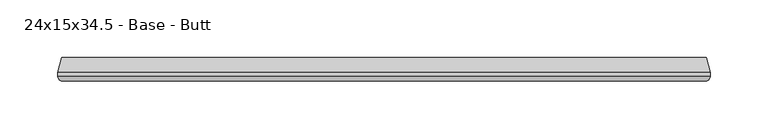
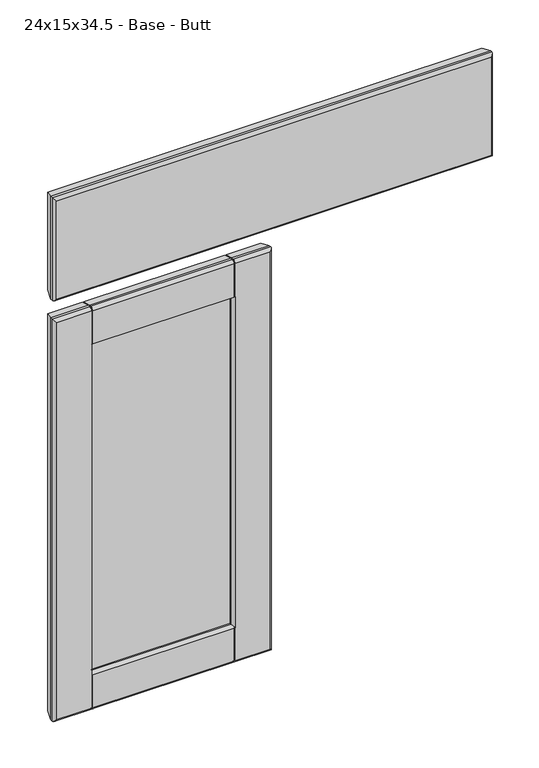
"""IFC4 building model written with IfcOpenShell, lengths in millimetres: furniture geometry, Cabinet-Base-Merillat-Double_Door-Marlin : 24x15x34.5 - Base - Butt."""

from ifc_helpers import new_model, si_unit, frame, origin, place, context, project, spatial, polyline, circle_curve, ellipse_curve, outline, extrude, source, transform, mapped, element, save
from ifc_brep_helpers import plane_surface, cylinder_surface, advanced_brep


def furniture_24x15x34_5_base_butt_84ca6513(model_context):
    return source(origin(), model_context, "Body", "SolidModel", [
        advanced_brep(
        [(-260.7408026, -629.92, 847.8035075), (-260.7408026, -629.92, 714.2964925), (298.2162124, -629.92, 714.2964925), (298.2162124, -629.92, 847.8035075), (-260.3320951, -609.6, 714.7052), (-260.3320951, -609.6, 847.3948), (297.8075049, -609.6, 847.3948), (297.8075049, -609.6, 714.7052), (-263.8372951, -625.4496, 850.9), (-263.8372951, -622.681, 850.9), (-263.8372951, -622.681, 711.2), (-263.8372951, -625.4496, 711.2), (301.3127049, -622.681, 711.2), (301.3127049, -625.4496, 711.2), (301.3127049, -622.681, 850.9), (301.3127049, -625.4496, 850.9)],
        [
            (0, 1),
            (1, 2),
            (2, 3),
            (3, 0),
            (4, 5),
            (5, 6),
            (6, 7),
            (7, 4),
            (8, 9),
            (9, 10),
            (10, 11),
            (11, 8),
            (10, 12),
            (12, 13),
            (13, 11),
            (12, 14),
            (14, 15),
            (15, 13),
            (8, 15),
            (14, 9),
            (11, 1, ellipse_curve(frame((-259.0620951, -625.4496, 715.9752), z_axis=(-0.7071067811865475, 0.0, 0.7071067811865475), x_axis=(-0.7071067811865474, 0.0, -0.7071067811865476)), 6.7531526, 4.7752)),
            (0, 8, ellipse_curve(frame((-259.0620951, -625.4496, 846.1248), z_axis=(-0.7071067811865475, 0.0, -0.7071067811865475), x_axis=(0.7071067811865474, 0.0, -0.7071067811865476)), 6.7531526, 4.7752)),
            (4, 10),
            (9, 5),
            (13, 2, ellipse_curve(frame((296.5375049, -625.4496, 715.9752), z_axis=(-0.7071067811865475, 0.0, -0.7071067811865475), x_axis=(0.7071067811865476, 0.0, -0.7071067811865474)), 6.7531526, 4.7752)),
            (7, 12),
            (15, 3, ellipse_curve(frame((296.5375049, -625.4496, 846.1248), z_axis=(0.7071067811865475, 0.0, -0.7071067811865475), x_axis=(0.7071067811865474, 0.0, 0.7071067811865476)), 6.7531526, 4.7752)),
            (6, 14),
        ],
        [
            plane_surface(frame((-263.8372951, -629.92, 850.9), z_axis=(0.0, -1.0, 0.0), x_axis=(0.0, 0.0, -1.0))),
            plane_surface(frame((-263.8372951, -609.6, 850.9), z_axis=(0.0, 1.0, 0.0), x_axis=(0.0, 0.0, 1.0))),
            plane_surface(frame((-263.8372951, -629.92, 850.9), z_axis=(-1.0, 0.0, 0.0), x_axis=(0.0, 1.0, 0.0))),
            plane_surface(frame((-263.8372951, -629.92, 711.2), z_axis=(0.0, 0.0, -1.0), x_axis=(0.0, 1.0, 0.0))),
            plane_surface(frame((301.3127049, -629.92, 711.2), z_axis=(1.0, 0.0, 0.0), x_axis=(0.0, 1.0, 0.0))),
            plane_surface(frame((301.3127049, -629.92, 850.9), z_axis=(0.0, 0.0, 1.0), x_axis=(0.0, 1.0, 0.0))),
            cylinder_surface(frame((-259.0620951, -625.4496, 850.9), z_axis=(0.0, 0.0, -1.0), x_axis=(0.0, 1.0, 0.0)), 4.7752),
            plane_surface(frame((-263.8372951, -622.681, 850.9), z_axis=(-0.9659229350723619, 0.25882983502910506, 0.0), x_axis=(0.0, 0.0, -1.0))),
            cylinder_surface(frame((-263.8372951, -625.4496, 715.9752), z_axis=(1.0, 0.0, 0.0), x_axis=(0.0, 1.0, 0.0)), 4.7752),
            plane_surface(frame((-263.8372951, -622.681, 711.2), z_axis=(0.0, 0.25882983502910506, -0.9659229350723619), x_axis=(1.0, 0.0, 0.0))),
            cylinder_surface(frame((296.5375049, -625.4496, 711.2), z_axis=(0.0, 0.0, 1.0), x_axis=(0.0, 1.0, 0.0)), 4.7752),
            plane_surface(frame((301.3127049, -622.681, 711.2), z_axis=(0.9659229350723619, 0.25882983502910506, 0.0), x_axis=(0.0, 0.0, 1.0))),
            cylinder_surface(frame((301.3127049, -625.4496, 846.1248), z_axis=(-1.0, 0.0, 0.0), x_axis=(0.0, 1.0, 0.0)), 4.7752),
            plane_surface(frame((301.3127049, -622.681, 850.9), z_axis=(0.0, 0.25882983502910506, 0.9659229350723619), x_axis=(-1.0, 0.0, 0.0))),
        ],
        [
            (0, [[1, 2, 3, 4]]),
            (1, [[5, 6, 7, 8]]),
            (2, [[9, 10, 11, 12]]),
            (3, [[-11, 13, 14, 15]]),
            (4, [[-14, 16, 17, 18]]),
            (5, [[-9, 19, -17, 20]]),
            (6, [[21, -1, 22, -12]]),
            (7, [[23, -10, 24, -5]]),
            (8, [[-21, -15, 25, -2]]),
            (9, [[-23, -8, 26, -13]]),
            (10, [[-25, -18, 27, -3]]),
            (11, [[-26, -7, 28, -16]]),
            (12, [[-22, -4, -27, -19]]),
            (13, [[-24, -20, -28, -6]]),
        ],
    ),
        advanced_brep(
        [(-263.8372951, -625.4496, 685.8), (-263.8372951, -625.4496, 139.7), (-260.7408026, -629.92, 142.7964925), (-260.7408026, -629.92, 682.7035075), (-263.8372951, -622.681, 685.8), (-263.8372951, -622.681, 139.7), (-260.3320951, -609.6, 682.2948), (-260.3320951, -609.6, 143.2052), (-215.6361323, -609.6, 637.5988372), (-215.2660006, -610.39375, 637.2287055), (-213.1848416, -614.85681, 635.1475465), (-213.1848416, -614.85681, 190.3524535), (-215.2660006, -610.39375, 188.2712945), (-215.6361323, -609.6, 187.9011628), (-214.584611, -617.0969093, 636.547316), (-214.584611, -617.0969093, 188.952684), (-228.9122951, -617.347, 650.875), (-228.9122951, -617.347, 174.625), (-228.9122951, -622.173, 650.875), (-228.9122951, -622.173, 174.625), (-214.584611, -622.4230907, 636.547316), (-214.584611, -622.4230907, 188.952684), (-213.1848416, -624.66319, 635.1475465), (-213.1848416, -624.66319, 190.3524535), (-215.2660006, -629.12625, 637.2287055), (-215.6332649, -629.9138508, 637.5959698), (-215.6361323, -629.92, 187.9011628), (-215.2660006, -629.12625, 188.2712945), (14.0537124, -629.92, 142.7964925), (-31.0140137, -629.92, 142.7964925), (-31.0140137, -625.4496, 139.7), (17.1502049, -625.4496, 139.7), (-215.6332649, -625.4496, 139.7), (-215.6332649, -629.92, 142.7964925), (-214.0457649, -625.4496, 139.7), (-32.6015137, -625.4496, 139.7), (-32.6015137, -629.92, 142.7964925), (-214.0457649, -629.92, 142.7964925), (-31.0140137, -622.681, 139.7), (17.1502049, -622.681, 139.7), (-215.6332649, -622.681, 139.7), (-214.0457649, -622.681, 139.7), (-32.6015137, -622.681, 139.7), (-31.0140137, -609.6, 143.2052), (13.6450049, -609.6, 143.2052), (-214.0457649, -609.6, 143.2052), (-32.6015137, -609.6, 143.2052), (-215.6332649, -609.6, 143.2052), (-33.5022486, -614.85681, 190.3524535), (-31.4210895, -610.39375, 188.2712945), (-32.6015137, -610.39375, 188.2712945), (-32.6015137, -609.6, 187.9011628), (-214.0457649, -609.6, 187.9011628), (-214.0457649, -610.39375, 188.2712945), (-32.1024791, -617.0969093, 188.952684), (-17.7747951, -617.347, 174.625), (-17.7747951, -622.173, 174.625), (-32.1024791, -622.4230907, 188.952684), (-33.5022486, -624.66319, 190.3524535), (-214.0457649, -629.12625, 188.2712945), (-214.0457649, -629.92, 187.9011628), (-32.6015137, -629.92, 187.9011628), (-32.6015137, -629.12625, 188.2712945), (-31.4210895, -629.12625, 188.2712945), (17.1502049, -625.4496, 685.8), (14.0537124, -629.92, 682.7035075), (17.1502049, -622.681, 685.8), (13.6450049, -609.6, 682.2948), (-31.0509578, -609.6, 187.9011628), (-33.5022486, -614.85681, 635.1475465), (-31.4210895, -610.39375, 637.2287055), (-31.0509578, -609.6, 637.5988372), (-32.1024791, -617.0969093, 636.547316), (-17.7747951, -617.347, 650.875), (-17.7747951, -622.173, 650.875), (-32.1024791, -622.4230907, 636.547316), (-33.5022486, -624.66319, 635.1475465), (-31.0509578, -629.92, 187.9011628), (-31.0509578, -629.92, 637.5988372), (-31.4210895, -629.12625, 637.2287055), (-215.6332649, -629.92, 682.7035075), (-215.6332649, -625.4496, 685.8), (-31.0140137, -625.4496, 685.8), (-31.0140137, -629.92, 682.7035075), (-32.6015137, -625.4496, 685.8), (-214.0457649, -625.4496, 685.8), (-214.0457649, -629.92, 682.7035075), (-32.6015137, -629.92, 682.7035075), (-215.6332649, -622.681, 685.8), (-31.0140137, -622.681, 685.8), (-32.6015137, -622.681, 685.8), (-214.0457649, -622.681, 685.8), (-215.6332649, -609.6, 682.2948), (-31.0140137, -609.6, 682.2948), (-32.6015137, -609.6, 682.2948), (-214.0457649, -609.6, 682.2948), (-32.6015137, -609.6, 637.5988372), (-214.0457649, -609.6, 637.5988372), (-214.0457649, -610.39375, 637.2287055), (-32.6015137, -610.39375, 637.2287055), (-32.6015137, -629.12625, 637.2287055), (-32.6015137, -629.92, 637.5988372), (-214.0457649, -629.92, 637.5988372), (-214.0457649, -629.12625, 637.2287055), (-32.6015137, -629.12625, 682.5526052), (-32.6015137, -625.4496, 685.00625), (-32.6015137, -622.7855037, 685.00625), (-32.6015137, -610.39375, 681.6857412), (-31.0140137, -610.39375, 637.2287055), (-31.0140137, -610.39375, 681.6857412), (-31.0140137, -622.7855037, 685.00625), (-31.0140137, -625.4496, 685.00625), (-31.0140137, -629.12625, 682.5526052), (-31.0140137, -629.12625, 637.2287055), (-215.6332649, -629.12625, 637.2287055), (-215.6332649, -629.12625, 682.5526052), (-215.6332649, -625.4496, 685.00625), (-215.6332649, -622.7855037, 685.00625), (-215.6332649, -610.39375, 681.6857412), (-215.6332649, -610.39375, 637.2287055), (-214.0457649, -610.39375, 681.6857412), (-214.0457649, -622.7855037, 685.00625), (-214.0457649, -625.4496, 685.00625), (-214.0457649, -629.12625, 682.5526052), (-215.6332649, -610.39375, 188.2712945), (-215.6332649, -610.39375, 143.8142588), (-215.6332649, -622.7855037, 140.49375), (-215.6332649, -625.4496, 140.49375), (-215.6332649, -629.12625, 142.9473948), (-215.6332649, -629.12625, 188.2712945), (-214.0457649, -629.12625, 142.9473948), (-214.0457649, -625.4496, 140.49375), (-214.0457649, -622.7855037, 140.49375), (-214.0457649, -610.39375, 143.8142588), (-32.6015137, -610.39375, 143.8142588), (-32.6015137, -622.7855037, 140.49375), (-32.6015137, -625.4496, 140.49375), (-32.6015137, -629.12625, 142.9473948), (-31.0140137, -629.12625, 188.2712945), (-31.0140137, -629.12625, 142.9473948), (-31.0140137, -625.4496, 140.49375), (-31.0140137, -622.7855037, 140.49375), (-31.0140137, -610.39375, 143.8142588), (-31.0140137, -610.39375, 188.2712945)],
        [
            (0, 1),
            (1, 2, ellipse_curve(frame((-259.0620951, -625.4496, 144.4752), z_axis=(-0.7071067811865475, 0.0, 0.7071067811865475), x_axis=(0.7071067811865474, 0.0, 0.7071067811865476)), 6.7531526, 4.7752)),
            (2, 3),
            (3, 0, ellipse_curve(frame((-259.0620951, -625.4496, 681.0248), z_axis=(-0.7071067811865475, 0.0, -0.7071067811865475), x_axis=(-0.7071067811865474, 0.0, 0.7071067811865476)), 6.7531526, 4.7752)),
            (0, 4),
            (4, 5),
            (5, 1),
            (4, 6),
            (6, 7),
            (7, 5),
            (8, 9),
            (9, 10),
            (10, 11),
            (11, 12),
            (12, 13),
            (13, 8),
            (10, 14, ellipse_curve(frame((-214.6120951, -615.5223492, 636.5748), z_axis=(-0.7071067811865475, 0.0, -0.7071067811865475), x_axis=(-0.7071067811865474, 0.0, 0.7071067811865476)), 2.2271035, 1.5748)),
            (14, 15),
            (15, 11, ellipse_curve(frame((-214.6120951, -615.5223492, 188.9252), z_axis=(-0.7071067811865475, 0.0, 0.7071067811865475), x_axis=(0.7071067811865474, 0.0, 0.7071067811865476)), 2.2271035, 1.5748)),
            (14, 16),
            (16, 17),
            (17, 15),
            (16, 18),
            (18, 19),
            (19, 17),
            (18, 20),
            (20, 21),
            (21, 19),
            (20, 22, ellipse_curve(frame((-214.6120951, -623.9976508, 636.5748), z_axis=(-0.7071067811865475, 0.0, -0.7071067811865475), x_axis=(-0.7071067811865474, 0.0, 0.7071067811865476)), 2.2271035, 1.5748)),
            (22, 23),
            (23, 21, ellipse_curve(frame((-214.6120951, -623.9976508, 188.9252), z_axis=(-0.7071067811865475, 0.0, 0.7071067811865475), x_axis=(0.7071067811865474, 0.0, 0.7071067811865476)), 2.2271035, 1.5748)),
            (22, 24),
            (24, 25),
            (25, 26),
            (26, 27),
            (27, 23),
            (28, 29),
            (29, 30, circle_curve(frame((-31.0140137, -625.4496, 144.4752), z_axis=(1.0, 0.0, 0.0), x_axis=(0.0, 1.0, 0.0)), 4.7752)),
            (30, 31),
            (31, 28, ellipse_curve(frame((12.3750049, -625.4496, 144.4752), z_axis=(-0.7071067811865475, 0.0, -0.7071067811865475), x_axis=(-0.7071067811865476, 0.0, 0.7071067811865474)), 6.7531526, 4.7752)),
            (1, 32),
            (32, 33, circle_curve(frame((-215.6332649, -625.4496, 144.4752), z_axis=(-1.0, 0.0, 0.0), x_axis=(0.0, 1.0, 0.0)), 4.7752)),
            (33, 2),
            (34, 35),
            (35, 36, circle_curve(frame((-32.6015137, -625.4496, 144.4752), z_axis=(-1.0, 0.0, 0.0), x_axis=(0.0, 1.0, 0.0)), 4.7752)),
            (36, 37),
            (37, 34, circle_curve(frame((-214.0457649, -625.4496, 144.4752), z_axis=(1.0, 0.0, 0.0), x_axis=(0.0, 1.0, 0.0)), 4.7752)),
            (30, 38),
            (38, 39),
            (39, 31),
            (5, 40),
            (40, 32),
            (41, 42),
            (42, 35),
            (34, 41),
            (38, 43),
            (43, 44),
            (44, 39),
            (45, 46),
            (46, 42),
            (41, 45),
            (7, 47),
            (47, 40),
            (48, 49),
            (49, 50),
            (50, 51),
            (51, 52),
            (52, 53),
            (53, 12),
            (11, 48),
            (15, 54),
            (54, 48, ellipse_curve(frame((-32.0749951, -615.5223492, 188.9252), z_axis=(-0.7071067811865475, 0.0, -0.7071067811865475), x_axis=(-0.7071067811865476, 0.0, 0.7071067811865474)), 2.2271035, 1.5748)),
            (17, 55),
            (55, 54),
            (19, 56),
            (56, 55),
            (21, 57),
            (57, 56),
            (23, 58),
            (58, 57, ellipse_curve(frame((-32.0749951, -623.9976508, 188.9252), z_axis=(-0.7071067811865475, 0.0, -0.7071067811865475), x_axis=(-0.7071067811865476, 0.0, 0.7071067811865474)), 2.2271035, 1.5748)),
            (27, 59),
            (59, 60),
            (60, 61),
            (61, 62),
            (62, 63),
            (63, 58),
            (31, 64),
            (64, 65, ellipse_curve(frame((12.3750049, -625.4496, 681.0248), z_axis=(0.7071067811865475, 0.0, -0.7071067811865475), x_axis=(-0.7071067811865474, 0.0, -0.7071067811865476)), 6.7531526, 4.7752)),
            (65, 28),
            (39, 66),
            (66, 64),
            (44, 67),
            (67, 66),
            (68, 49),
            (48, 69),
            (69, 70),
            (70, 71),
            (71, 68),
            (54, 72),
            (72, 69, ellipse_curve(frame((-32.0749951, -615.5223492, 636.5748), z_axis=(0.7071067811865475, 0.0, -0.7071067811865475), x_axis=(-0.7071067811865474, 0.0, -0.7071067811865476)), 2.2271035, 1.5748)),
            (55, 73),
            (73, 72),
            (56, 74),
            (74, 73),
            (57, 75),
            (75, 74),
            (58, 76),
            (76, 75, ellipse_curve(frame((-32.0749951, -623.9976508, 636.5748), z_axis=(0.7071067811865475, 0.0, -0.7071067811865475), x_axis=(-0.7071067811865474, 0.0, -0.7071067811865476)), 2.2271035, 1.5748)),
            (63, 77),
            (77, 78),
            (78, 79),
            (79, 76),
            (3, 80),
            (80, 81, circle_curve(frame((-215.6332649, -625.4496, 681.0248), z_axis=(-1.0, 0.0, 0.0), x_axis=(0.0, 1.0, 0.0)), 4.7752)),
            (81, 0),
            (64, 82),
            (82, 83, circle_curve(frame((-31.0140137, -625.4496, 681.0248), z_axis=(1.0, 0.0, 0.0), x_axis=(0.0, 1.0, 0.0)), 4.7752)),
            (83, 65),
            (84, 85),
            (85, 86, circle_curve(frame((-214.0457649, -625.4496, 681.0248), z_axis=(1.0, 0.0, 0.0), x_axis=(0.0, 1.0, 0.0)), 4.7752)),
            (86, 87),
            (87, 84, circle_curve(frame((-32.6015137, -625.4496, 681.0248), z_axis=(-1.0, 0.0, 0.0), x_axis=(0.0, 1.0, 0.0)), 4.7752)),
            (81, 88),
            (88, 4),
            (66, 89),
            (89, 82),
            (90, 91),
            (91, 85),
            (84, 90),
            (88, 92),
            (92, 6),
            (67, 93),
            (93, 89),
            (94, 95),
            (95, 91),
            (90, 94),
            (51, 46),
            (45, 52),
            (43, 68),
            (71, 93),
            (92, 8),
            (13, 47),
            (96, 97),
            (97, 95),
            (94, 96),
            (9, 98),
            (98, 97),
            (96, 99),
            (99, 70),
            (69, 10),
            (72, 14),
            (73, 16),
            (74, 18),
            (75, 20),
            (76, 22),
            (79, 100),
            (100, 101),
            (101, 102),
            (102, 103),
            (103, 24),
            (33, 26),
            (25, 80),
            (36, 61),
            (60, 37),
            (83, 78),
            (77, 29),
            (86, 102),
            (101, 87),
            (100, 104),
            (104, 105, circle_curve(frame((-32.6015137, -625.4496, 681.0248), z_axis=(-1.0, 0.0, 0.0), x_axis=(0.0, 0.0, 1.0)), 3.98145)),
            (105, 106),
            (106, 107),
            (107, 99),
            (71, 108),
            (108, 109),
            (109, 110),
            (110, 111),
            (111, 112, circle_curve(frame((-31.0140137, -625.4496, 681.0248), z_axis=(1.0, 0.0, 0.0), x_axis=(0.0, 0.0, 1.0)), 3.98145)),
            (112, 113),
            (113, 78),
            (113, 79),
            (112, 104),
            (111, 105),
            (110, 106),
            (109, 107),
            (108, 70),
            (25, 114),
            (114, 115),
            (115, 116, circle_curve(frame((-215.6332649, -625.4496, 681.0248), z_axis=(-1.0, 0.0, 0.0), x_axis=(0.0, 0.0, 1.0)), 3.98145)),
            (116, 117),
            (117, 118),
            (118, 119),
            (119, 8),
            (98, 120),
            (120, 121),
            (121, 122),
            (122, 123, circle_curve(frame((-214.0457649, -625.4496, 681.0248), z_axis=(1.0, 0.0, 0.0), x_axis=(0.0, 0.0, 1.0)), 3.98145)),
            (123, 103),
            (24, 114),
            (123, 115),
            (122, 116),
            (121, 117),
            (120, 118),
            (9, 119),
            (13, 124),
            (124, 125),
            (125, 126),
            (126, 127),
            (127, 128, circle_curve(frame((-215.6332649, -625.4496, 144.4752), z_axis=(-1.0, 0.0, 0.0), x_axis=(0.0, 0.0, 1.0)), 3.98145)),
            (128, 129),
            (129, 26),
            (59, 130),
            (130, 131, circle_curve(frame((-214.0457649, -625.4496, 144.4752), z_axis=(1.0, 0.0, 0.0), x_axis=(0.0, 0.0, 1.0)), 3.98145)),
            (131, 132),
            (132, 133),
            (133, 53),
            (12, 124),
            (133, 125),
            (132, 126),
            (131, 127),
            (130, 128),
            (27, 129),
            (50, 134),
            (134, 135),
            (135, 136),
            (136, 137, circle_curve(frame((-32.6015137, -625.4496, 144.4752), z_axis=(-1.0, 0.0, 0.0), x_axis=(0.0, 0.0, 1.0)), 3.98145)),
            (137, 62),
            (138, 139),
            (139, 140, circle_curve(frame((-31.0140137, -625.4496, 144.4752), z_axis=(1.0, 0.0, 0.0), x_axis=(0.0, 0.0, 1.0)), 3.98145)),
            (140, 141),
            (141, 142),
            (142, 143),
            (143, 68),
            (77, 138),
            (63, 138),
            (143, 49),
            (142, 134),
            (141, 135),
            (140, 136),
            (139, 137),
        ],
        [
            cylinder_surface(frame((-259.0620951, -625.4496, 685.8), z_axis=(0.0, 0.0, 1.0), x_axis=(0.0, 1.0, 0.0)), 4.7752),
            plane_surface(frame((-263.8372951, -625.4496, 685.8), z_axis=(-1.0, 0.0, 0.0), x_axis=(0.0, 0.0, -1.0))),
            plane_surface(frame((-263.8372951, -622.681, 685.8), z_axis=(-0.9659229350723619, 0.25882983502910506, 0.0), x_axis=(0.0, 0.0, -1.0))),
            plane_surface(frame((-215.6361323, -609.6, 637.5988372), z_axis=(0.9063077870366099, 0.4226182617407856, 0.0), x_axis=(0.0, 0.0, -1.0))),
            cylinder_surface(frame((-214.6120951, -615.5223492, 685.8), z_axis=(0.0, 0.0, 1.0000000000000002), x_axis=(0.01745240643729364, -0.9998476951563912, 0.0)), 1.5748),
            plane_surface(frame((-214.584611, -617.0969093, 636.547316), z_axis=(0.017452406437322144, -0.9998476951563906, 0.0), x_axis=(0.0, 0.0, -1.0))),
            plane_surface(frame((-228.9122951, -617.347, 650.875), z_axis=(1.0, 0.0, 0.0), x_axis=(0.0, 0.0, -1.0))),
            plane_surface(frame((-228.9122951, -622.173, 650.875), z_axis=(0.01745240643727848, 0.9998476951563914, 0.0), x_axis=(0.0, 0.0, -1.0))),
            cylinder_surface(frame((-214.6120951, -623.9976508, 685.8), z_axis=(0.0, 0.0, 1.0000000000000002), x_axis=(0.9063077870367326, -0.42261826174052236, 0.0)), 1.5748),
            plane_surface(frame((-213.1848416, -624.66319, 635.1475465), z_axis=(0.9063077870366333, -0.4226182617407352, 0.0), x_axis=(0.0, 0.0, -1.0))),
            cylinder_surface(frame((-263.8372951, -625.4496, 144.4752), z_axis=(-1.0, 0.0, 0.0), x_axis=(0.0, 1.0, 0.0)), 4.7752),
            plane_surface(frame((-263.8372951, -625.4496, 139.7), z_axis=(0.0, 0.0, -1.0), x_axis=(1.0, 0.0, 0.0))),
            plane_surface(frame((-263.8372951, -622.681, 139.7), z_axis=(0.0, 0.25882983502910506, -0.9659229350723619), x_axis=(1.0, 0.0, 0.0))),
            plane_surface(frame((-215.6361323, -609.6, 187.9011628), z_axis=(0.0, 0.4226182617407856, 0.9063077870366099), x_axis=(1.0, 0.0, 0.0))),
            cylinder_surface(frame((-263.8372951, -615.5223492, 188.9252), z_axis=(-1.0000000000000002, 0.0, 0.0), x_axis=(0.0, -0.9998476951563912, 0.01745240643729364)), 1.5748),
            plane_surface(frame((-214.584611, -617.0969093, 188.952684), z_axis=(0.0, -0.9998476951563906, 0.017452406437322144), x_axis=(1.0, 0.0, 0.0))),
            plane_surface(frame((-228.9122951, -617.347, 174.625), z_axis=(0.0, 0.0, 1.0), x_axis=(1.0, 0.0, 0.0))),
            plane_surface(frame((-228.9122951, -622.173, 174.625), z_axis=(0.0, 0.9998476951563914, 0.01745240643727848), x_axis=(1.0, 0.0, 0.0))),
            cylinder_surface(frame((-263.8372951, -623.9976508, 188.9252), z_axis=(-1.0000000000000002, 0.0, 0.0), x_axis=(0.0, -0.42261826174052236, 0.9063077870367326)), 1.5748),
            plane_surface(frame((-213.1848416, -624.66319, 190.3524535), z_axis=(0.0, -0.4226182617407352, 0.9063077870366333), x_axis=(1.0, 0.0, 0.0))),
            cylinder_surface(frame((12.3750049, -625.4496, 139.7), z_axis=(0.0, 0.0, -1.0), x_axis=(0.0, 1.0, 0.0)), 4.7752),
            plane_surface(frame((17.1502049, -625.4496, 139.7), z_axis=(1.0, 0.0, 0.0), x_axis=(0.0, 0.0, 1.0))),
            plane_surface(frame((17.1502049, -622.681, 139.7), z_axis=(0.9659229350723619, 0.25882983502910506, 0.0), x_axis=(0.0, 0.0, 1.0))),
            plane_surface(frame((-31.0509578, -609.6, 187.9011628), z_axis=(-0.9063077870366099, 0.4226182617407856, 0.0), x_axis=(0.0, 0.0, 1.0))),
            cylinder_surface(frame((-32.0749951, -615.5223492, 139.7), z_axis=(0.0, 0.0, -1.0000000000000002), x_axis=(-0.01745240643729364, -0.9998476951563912, 0.0)), 1.5748),
            plane_surface(frame((-32.1024791, -617.0969093, 188.952684), z_axis=(-0.017452406437322144, -0.9998476951563906, 0.0), x_axis=(0.0, 0.0, 1.0))),
            plane_surface(frame((-17.7747951, -617.347, 174.625), z_axis=(-1.0, 0.0, 0.0), x_axis=(0.0, 0.0, 1.0))),
            plane_surface(frame((-17.7747951, -622.173, 174.625), z_axis=(-0.01745240643727848, 0.9998476951563914, 0.0), x_axis=(0.0, 0.0, 1.0))),
            cylinder_surface(frame((-32.0749951, -623.9976508, 139.7), z_axis=(0.0, 0.0, -1.0000000000000002), x_axis=(-0.9063077870367326, -0.42261826174052236, 0.0)), 1.5748),
            plane_surface(frame((-33.5022486, -624.66319, 190.3524535), z_axis=(-0.9063077870366333, -0.4226182617407352, 0.0), x_axis=(0.0, 0.0, 1.0))),
            cylinder_surface(frame((17.1502049, -625.4496, 681.0248), z_axis=(1.0, 0.0, 0.0), x_axis=(0.0, 1.0, 0.0)), 4.7752),
            plane_surface(frame((17.1502049, -625.4496, 685.8), z_axis=(0.0, 0.0, 1.0), x_axis=(-1.0, 0.0, 0.0))),
            plane_surface(frame((17.1502049, -622.681, 685.8), z_axis=(0.0, 0.25882983502910506, 0.9659229350723619), x_axis=(-1.0, 0.0, 0.0))),
            plane_surface(frame((13.6450049, -609.6, 682.2948), z_axis=(0.0, 1.0, 0.0), x_axis=(-1.0, 0.0, 0.0))),
            plane_surface(frame((-31.0509578, -609.6, 637.5988372), z_axis=(0.0, 0.4226182617407856, -0.9063077870366099), x_axis=(-1.0, 0.0, 0.0))),
            cylinder_surface(frame((17.1502049, -615.5223492, 636.5748), z_axis=(1.0000000000000002, 0.0, 0.0), x_axis=(0.0, -0.9998476951563912, -0.01745240643729364)), 1.5748),
            plane_surface(frame((-32.1024791, -617.0969093, 636.547316), z_axis=(0.0, -0.9998476951563906, -0.017452406437322144), x_axis=(-1.0, 0.0, 0.0))),
            plane_surface(frame((-17.7747951, -617.347, 650.875), z_axis=(0.0, 0.0, -1.0), x_axis=(-1.0, 0.0, 0.0))),
            plane_surface(frame((-17.7747951, -622.173, 650.875), z_axis=(0.0, 0.9998476951563914, -0.01745240643727848), x_axis=(-1.0, 0.0, 0.0))),
            cylinder_surface(frame((17.1502049, -623.9976508, 636.5748), z_axis=(1.0000000000000002, 0.0, 0.0), x_axis=(0.0, -0.42261826174052236, -0.9063077870367326)), 1.5748),
            plane_surface(frame((-33.5022486, -624.66319, 635.1475465), z_axis=(0.0, -0.4226182617407352, -0.9063077870366333), x_axis=(-1.0, 0.0, 0.0))),
            plane_surface(frame((-31.0509578, -629.92, 637.5988372), z_axis=(0.0, -1.0, 0.0), x_axis=(-1.0, 0.0, 0.0))),
            plane_surface(frame((-32.6015137, -629.92, 637.5988372), z_axis=(1.0, 0.0, 0.0), x_axis=(0.0, 0.906307787036771, -0.4226182617404399))),
            plane_surface(frame((-31.0140137, -629.92, 637.5988372), z_axis=(-1.0, 0.0, 0.0), x_axis=(0.0, -0.906307787036771, 0.4226182617404399))),
            plane_surface(frame((-32.6015137, -629.92, 637.5988372), z_axis=(0.0, 0.4226182617404399, 0.906307787036771), x_axis=(1.0, 0.0, 0.0))),
            plane_surface(frame((-32.6015137, -629.12625, 637.2287055), z_axis=(0.0, -1.0, 0.0), x_axis=(1.0, 0.0, 0.0))),
            cylinder_surface(frame((-31.0140137, -625.4496, 681.0248), z_axis=(1.0, 0.0, 0.0), x_axis=(0.0, 0.0, 1.0)), 3.98145),
            plane_surface(frame((-32.6015137, -625.4496, 685.00625), z_axis=(0.0, 0.0, 1.0), x_axis=(1.0, 0.0, 0.0))),
            plane_surface(frame((-32.6015137, -622.7855037, 685.00625), z_axis=(0.0, 0.25882983502913415, 0.9659229350723542), x_axis=(1.0, 0.0, 0.0))),
            plane_surface(frame((-32.6015137, -610.39375, 681.6857412), z_axis=(0.0, 1.0, 0.0), x_axis=(1.0, 0.0, 0.0))),
            plane_surface(frame((-32.6015137, -610.39375, 637.2287055), z_axis=(0.0, -0.4226182617405111, 0.9063077870367379), x_axis=(1.0, 0.0, 0.0))),
            plane_surface(frame((-215.6332649, -629.92, 637.5988372), z_axis=(1.0, 0.0, 0.0), x_axis=(0.0, 0.9063077870367783, -0.42261826174042444))),
            plane_surface(frame((-214.0457649, -629.92, 637.5988372), z_axis=(-1.0, 0.0, 0.0), x_axis=(0.0, -0.9063077870367783, 0.42261826174042444))),
            plane_surface(frame((-215.6332649, -629.92, 637.5988372), z_axis=(0.0, 0.42261826174042444, 0.9063077870367783), x_axis=(1.0, 0.0, 0.0))),
            plane_surface(frame((-215.6332649, -629.12625, 637.2287055), z_axis=(0.0, -1.0, 0.0), x_axis=(1.0, 0.0, 0.0))),
            cylinder_surface(frame((-214.0457649, -625.4496, 681.0248), z_axis=(1.0, 0.0, 0.0), x_axis=(0.0, 0.0, 1.0)), 3.98145),
            plane_surface(frame((-215.6332649, -625.4496, 685.00625), z_axis=(0.0, 0.0, 1.0), x_axis=(1.0, 0.0, 0.0))),
            plane_surface(frame((-215.6332649, -622.7855037, 685.00625), z_axis=(0.0, 0.25882983502911566, 0.965922935072359), x_axis=(1.0, 0.0, 0.0))),
            plane_surface(frame((-215.6332649, -610.39375, 681.6857412), z_axis=(0.0, 1.0, 0.0), x_axis=(1.0, 0.0, 0.0))),
            plane_surface(frame((-215.6332649, -610.39375, 637.2287055), z_axis=(0.0, -0.42261826174056427, 0.9063077870367131), x_axis=(1.0, 0.0, 0.0))),
            plane_surface(frame((-215.6332649, -625.4496, 149.2504), z_axis=(1.0, 0.0, 0.0), x_axis=(0.0, -1.0, 0.0))),
            plane_surface(frame((-214.0457649, -625.4496, 149.2504), z_axis=(-1.0, 0.0, 0.0), x_axis=(0.0, 1.0, 0.0))),
            plane_surface(frame((-215.6332649, -609.6, 187.9011628), z_axis=(0.0, -0.42261826173999295, -0.9063077870369795), x_axis=(1.0, 0.0, 0.0))),
            plane_surface(frame((-215.6332649, -610.39375, 188.2712945), z_axis=(0.0, 1.0, 0.0), x_axis=(1.0, 0.0, 0.0))),
            plane_surface(frame((-215.6332649, -610.39375, 143.8142588), z_axis=(0.0, 0.2588298350290845, -0.9659229350723675), x_axis=(1.0, 0.0, 0.0))),
            plane_surface(frame((-215.6332649, -622.7855037, 140.49375), z_axis=(0.0, 0.0, -1.0), x_axis=(1.0, 0.0, 0.0))),
            cylinder_surface(frame((-214.0457649, -625.4496, 144.4752), z_axis=(1.0, 0.0, 0.0), x_axis=(0.0, 0.0, 1.0)), 3.98145),
            plane_surface(frame((-215.6332649, -629.12625, 142.9473948), z_axis=(0.0, -1.0, 0.0), x_axis=(1.0, 0.0, 0.0))),
            plane_surface(frame((-215.6332649, -629.12625, 188.2712945), z_axis=(0.0, 0.4226182617407698, -0.9063077870366172), x_axis=(1.0, 0.0, 0.0))),
            plane_surface(frame((-32.6015137, -629.12625, 188.2712945), z_axis=(1.0, 0.0, 0.0), x_axis=(0.0, -0.906307787036583, -0.42261826174084305))),
            plane_surface(frame((-31.0140137, -629.12625, 188.2712945), z_axis=(-1.0, 0.0, 0.0), x_axis=(0.0, 0.906307787036583, 0.42261826174084305))),
            plane_surface(frame((-32.6015137, -629.12625, 188.2712945), z_axis=(0.0, 0.42261826174084305, -0.906307787036583), x_axis=(1.0, 0.0, 0.0))),
            plane_surface(frame((-32.6015137, -609.6, 187.9011628), z_axis=(0.0, -0.42261826174073325, -0.9063077870366342), x_axis=(1.0, 0.0, 0.0))),
            plane_surface(frame((-32.6015137, -610.39375, 188.2712945), z_axis=(0.0, 1.0, 0.0), x_axis=(1.0, 0.0, 0.0))),
            plane_surface(frame((-32.6015137, -610.39375, 143.8142588), z_axis=(0.0, 0.2588298350290967, -0.9659229350723642), x_axis=(1.0, 0.0, 0.0))),
            plane_surface(frame((-32.6015137, -622.7855037, 140.49375), z_axis=(0.0, 0.0, -1.0), x_axis=(1.0, 0.0, 0.0))),
            cylinder_surface(frame((-31.0140137, -625.4496, 144.4752), z_axis=(1.0, 0.0, 0.0), x_axis=(0.0, 0.0, 1.0)), 3.98145),
            plane_surface(frame((-32.6015137, -629.12625, 142.9473948), z_axis=(0.0, -1.0, 0.0), x_axis=(1.0, 0.0, 0.0))),
        ],
        [
            (0, [[1, 2, 3, 4]]),
            (1, [[5, 6, 7, -1]]),
            (2, [[8, 9, 10, -6]]),
            (3, [[11, 12, 13, 14, 15, 16]]),
            (4, [[17, 18, 19, -13]]),
            (5, [[20, 21, 22, -18]]),
            (6, [[23, 24, 25, -21]]),
            (7, [[26, 27, 28, -24]]),
            (8, [[29, 30, 31, -27]]),
            (9, [[32, 33, 34, 35, 36, -30]]),
            (10, [[37, 38, 39, 40]]),
            (10, [[41, 42, 43, -2]]),
            (10, [[44, 45, 46, 47]]),
            (11, [[-39, 48, 49, 50]]),
            (11, [[51, 52, -41, -7]]),
            (11, [[53, 54, -44, 55]]),
            (12, [[-49, 56, 57, 58]]),
            (12, [[59, 60, -53, 61]]),
            (12, [[62, 63, -51, -10]]),
            (13, [[64, 65, 66, 67, 68, 69, -14, 70]]),
            (14, [[71, 72, -70, -19]]),
            (15, [[73, 74, -71, -22]]),
            (16, [[75, 76, -73, -25]]),
            (17, [[77, 78, -75, -28]]),
            (18, [[79, 80, -77, -31]]),
            (19, [[-36, 81, 82, 83, 84, 85, 86, -79]]),
            (20, [[87, 88, 89, -40]]),
            (21, [[90, 91, -87, -50]]),
            (22, [[92, 93, -90, -58]]),
            (23, [[94, -64, 95, 96, 97, 98]]),
            (24, [[99, 100, -95, -72]]),
            (25, [[101, 102, -99, -74]]),
            (26, [[103, 104, -101, -76]]),
            (27, [[105, 106, -103, -78]]),
            (28, [[107, 108, -105, -80]]),
            (29, [[-86, 109, 110, 111, 112, -107]]),
            (30, [[113, 114, 115, -4]]),
            (30, [[116, 117, 118, -88]]),
            (30, [[119, 120, 121, 122]]),
            (31, [[-115, 123, 124, -5]]),
            (31, [[125, 126, -116, -91]]),
            (31, [[127, 128, -119, 129]]),
            (32, [[-124, 130, 131, -8]]),
            (32, [[132, 133, -125, -93]]),
            (32, [[134, 135, -127, 136]]),
            (33, [[-67, 137, -59, 138]]),
            (33, [[-57, 139, -98, 140, -132, -92]]),
            (33, [[-131, 141, -16, 142, -62, -9]]),
            (33, [[143, 144, -134, 145]]),
            (34, [[-12, 146, 147, -143, 148, 149, -96, 150]]),
            (35, [[-150, -100, 151, -17]]),
            (36, [[-151, -102, 152, -20]]),
            (37, [[-152, -104, 153, -23]]),
            (38, [[-153, -106, 154, -26]]),
            (39, [[-154, -108, 155, -29]]),
            (40, [[-112, 156, 157, 158, 159, 160, -32, -155]]),
            (41, [[-43, 161, -34, 162, -113, -3]]),
            (41, [[-46, 163, -83, 164]]),
            (41, [[-118, 165, -110, 166, -37, -89]]),
            (41, [[-121, 167, -158, 168]]),
            (42, [[-148, -145, -136, -129, -122, -168, -157, 169, 170, 171, 172, 173]]),
            (43, [[-165, -117, -126, -133, -140, 174, 175, 176, 177, 178, 179, 180]]),
            (44, [[181, -111, -180]]),
            (45, [[-156, -181, -179, 182, -169]]),
            (46, [[-182, -178, 183, -170]]),
            (47, [[-183, -177, 184, -171]]),
            (48, [[-184, -176, 185, -172]]),
            (49, [[-185, -175, 186, -149, -173]]),
            (50, [[-97, -186, -174]]),
            (51, [[-141, -130, -123, -114, -162, 187, 188, 189, 190, 191, 192, 193]]),
            (52, [[-159, -167, -120, -128, -135, -144, -147, 194, 195, 196, 197, 198]]),
            (53, [[-33, 199, -187]]),
            (54, [[-199, -160, -198, 200, -188]]),
            (55, [[-200, -197, 201, -189]]),
            (56, [[-201, -196, 202, -190]]),
            (57, [[-202, -195, 203, -191]]),
            (58, [[-203, -194, -146, 204, -192]]),
            (59, [[-204, -11, -193]]),
            (60, [[-161, -42, -52, -63, -142, 205, 206, 207, 208, 209, 210, 211]]),
            (61, [[-68, -138, -61, -55, -47, -164, -82, 212, 213, 214, 215, 216]]),
            (62, [[-15, 217, -205]]),
            (63, [[-217, -69, -216, 218, -206]]),
            (64, [[-218, -215, 219, -207]]),
            (65, [[-219, -214, 220, -208]]),
            (66, [[-220, -213, 221, -209]]),
            (67, [[-221, -212, -81, 222, -210]]),
            (68, [[-222, -35, -211]]),
            (69, [[-84, -163, -45, -54, -60, -137, -66, 223, 224, 225, 226, 227]]),
            (70, [[228, 229, 230, 231, 232, 233, -139, -56, -48, -38, -166, 234]]),
            (71, [[-109, 235, -234]]),
            (72, [[236, -94, -233]]),
            (73, [[-65, -236, -232, 237, -223]]),
            (74, [[-237, -231, 238, -224]]),
            (75, [[-238, -230, 239, -225]]),
            (76, [[-239, -229, 240, -226]]),
            (77, [[-240, -228, -235, -85, -227]]),
        ],
    ),
        extrude(outline(polyline([(-17.7747951, -622.173), (-228.9122951, -622.173), (-228.9122951, -617.347), (-17.7747951, -617.347), (-17.7747951, -622.173)])), frame((0.0, 0.0, 174.625), z_axis=(0.0, 0.0, 1.0), x_axis=(1.0, 0.0, 0.0)), (0.0, 0.0, 1.0), 476.25),
    ])


if __name__ == "__main__":
    model = new_model("IFC4")
    model_context = context("Model", 3, world=origin())
    ifc_project = project(units=[si_unit("LENGTHUNIT", "METRE", prefix="MILLI")], contexts=[model_context])
    site = spatial("IfcSite", under=ifc_project)
    building = spatial("IfcBuilding", under=site)
    placement = place(None, origin())
    furniture_24x15x34_5_base_butt_shape = furniture_24x15x34_5_base_butt_84ca6513(model_context)
    element("IfcFurniture", 1, ObjectType="Cabinet-Base-Merillat-Double_Door-Marlin : 24x15x34.5 - Base - Butt", at=placement, inside=building, context=model_context, shape_type="MappedRepresentation", body=[
        mapped(furniture_24x15x34_5_base_butt_shape, transform((0.0, 0.0, 0.0), x_axis=(1.0, 0.0, 0.0), y_axis=(0.0, 1.0, 0.0), z_axis=(0.0, 0.0, 1.0))),
    ])
    save(model, "model.ifc")

# Revit data of these elements
# Type "Cabinet-Base-Merillat-Double_Door-Marlin : 24x15x34.5 - Base - Butt"
#   URL = "http://www.merillat.com"
#   Toe Kick Note = "Toe Kick Covering is not included. To be purchased Separately."
#   Product Line = "Express"
#   Product Page URL = "http://www.merillat.com//our-products/rooms/kitchen"
#   Product Group = "Base Cabinet"
#   Product Documentation Link = "http://merillatbusiness.com/customer-resources/product-line-resources/merillat-classic/"
#   Model = "B24B"
#   Manufacturer = "Merillat"
#   Finish = "Wood"
#   Description = "Base Butt Door"
#   Construction Type = "Deep Sink Base"
#   Cabinet Construction Note = "BUTT doors without a center frame stile, For tray or shelf option,  replace HDS with the option code of your choice,  When depth is reduced  to 12\" or 15\" drawer becomes false front"
#   Assembly Code = "C1030410"
#   Toe Kick Height = 0' - 4 1/2"
#   Toe Kick Depth = 0' - 2 25/32"
#   Top and Bottom Spacing = 0' - 1"
#   Side Spacing = 0' - 0 7/8"
#   Cabinet Shell = 0' - 0 3/8"
#   Door Spacing = 0' - 0 1/8"
#   Depth = 1' - 3"
#   Height = 2' - 10 1/2"
#   Width = 2' - 0"
#   Cabinet Drawer Width = 1' - 10 1/4"
#   Cabinet Drawer Height = 0' - 5 1/2"
#   Cabinet Drawer 2 Drawer Width = 0' - 11 1/16"
#   Cabinet Door Width = 0' - 11 1/16"
#   Cabinet Door Height = 1' - 9 1/2"
#   COBie.Type = no
#   Two Drawer = no
#   Elevation Swing Line = yes
#   Partial Overlay = yes
#   One Drawer = yes
#   Full Overlay = no
#   Butt Option = yes
#   Toe Kick Material = Wood - Merillat - Raw Particle Board
#   Door Drawer Material = Wood - Merillat - Pecan(1)
#   Cabinet Material = Wood - Merillat - Pecan(1)
#   Cabinet Drawer Style 2 Drawer = element 819256
#   Cabinet Drawer Style = element 819255
#   Cabinet Door Style = element 819254
# Element 1 (IfcFurniture, "Cabinet-Base-Merillat-Double_Door-Marlin : 24x15x34.5 - Base - Butt")
#   Materials on its faces: "Wood - Merillat - Pecan(1)", "Wood - Merillat - Raw Particle Board"
# Materials
#   "Wood - Merillat - Raw Particle Board": class "Plastic", colour RGB 80 80 80, transparency 0, Description = "Plastic Laminate - Navy", Cost = 0
#   "Wood - Merillat - Pecan(1)": class "Wood", colour RGB 108 67 43, transparency 0, Cost = 0
